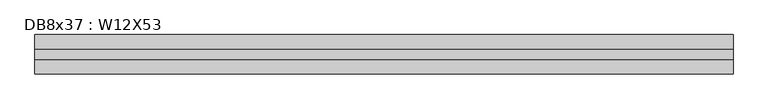
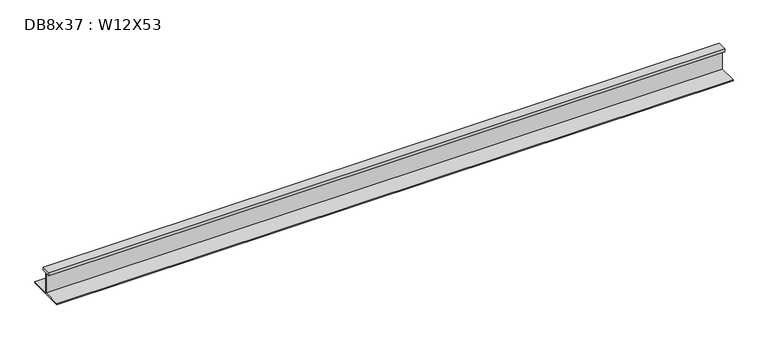
"""IFC4 building model written with IfcOpenShell, lengths in millimetres: beam geometry, DB8x37 : W12X53."""

from ifc_helpers import new_model, si_unit, frame, origin, place, context, project, spatial, polyline, outline, extrude, source, transform, mapped, element, save


def db8x37_w12x53_103d37c9(model_context):
    return source(origin(), model_context, "Body", "SweptSolid", [
        extrude(outline(polyline([(38.1, 145.415), (38.1, 120.015), (2.921, 120.015), (2.921, -48.4505), (152.4, -48.4505), (152.4, -58.1025), (-152.4, -58.1025), (-152.4, -48.4505), (-2.921, -48.4505), (-2.921, 120.015), (-38.1, 120.015), (-38.1, 145.415), (38.1, 145.415)])), frame((-2708.529, 0.0, 0.0), z_axis=(1.0, 0.0, 0.0), x_axis=(0.0, 1.0, 0.0)), (0.0, 0.0, 1.0), 5389.499),
    ])


if __name__ == "__main__":
    model = new_model("IFC4")
    model_context = context("Model", 3, world=origin())
    ifc_project = project(units=[si_unit("LENGTHUNIT", "METRE", prefix="MILLI")], contexts=[model_context])
    site = spatial("IfcSite", under=ifc_project)
    building = spatial("IfcBuilding", under=site)
    placement = place(None, origin())
    db8x37_w12x53_shape = db8x37_w12x53_103d37c9(model_context)
    element("IfcBeam", 1, ObjectType="DB8x37 : W12X53", at=placement, inside=building, context=model_context, shape_type="MappedRepresentation", body=[
        mapped(db8x37_w12x53_shape, transform((0.0, 0.0, 0.0), x_axis=(1.0, 0.0, 0.0), y_axis=(0.0, 1.0, 0.0), z_axis=(0.0, 0.0, 1.0))),
    ])
    save(model, "model.ifc")

# Revit data of these elements
# Type "DB8x37 : W12X53"
#   Assembly Code = "B10"
#   W = 53
#   Length [instance default] = 5' - 0"
#   bf = 0' - 10"
#   d = 1' - 0.1"
#   k = 0' - 1 3/8"
#   k2 = 0' - 0.8"
#   tf = 0' - 0.575"
#   tw = 0' - 0.345"
#   A = 0.108333 SF
#   Structural Material [instance default] = Steel ASTM A992
# Element 1 (IfcBeam, "DB8x37 : W12X53")
#   Materials on its faces: "Steel ASTM A992"
# Materials
#   "Steel ASTM A992": class "Metal", colour RGB 199 199 199, transparency 0, Description = "Structural steel 50ksi", Cost = 0
